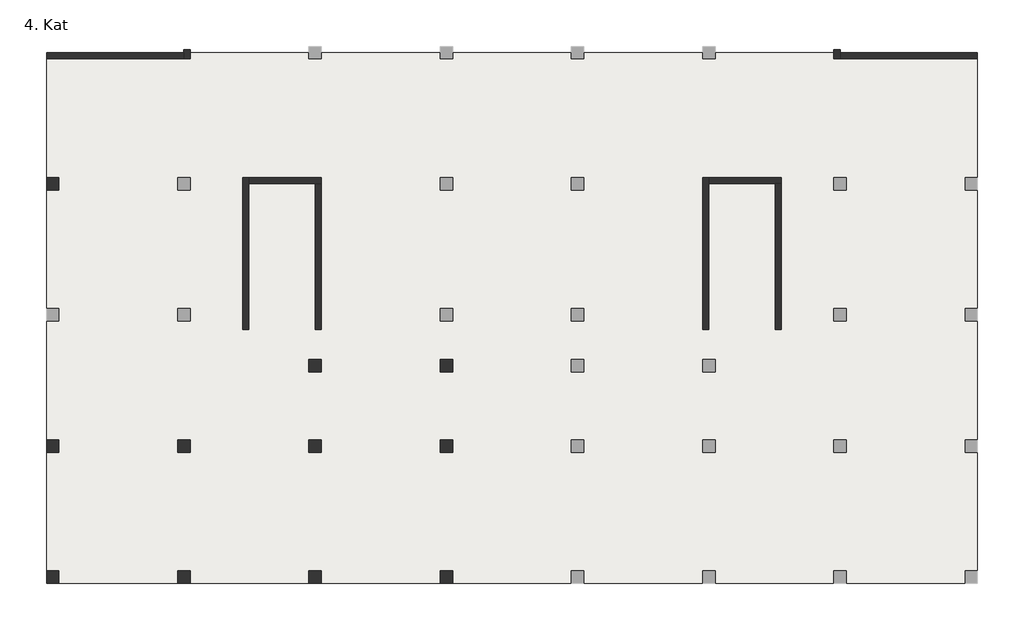
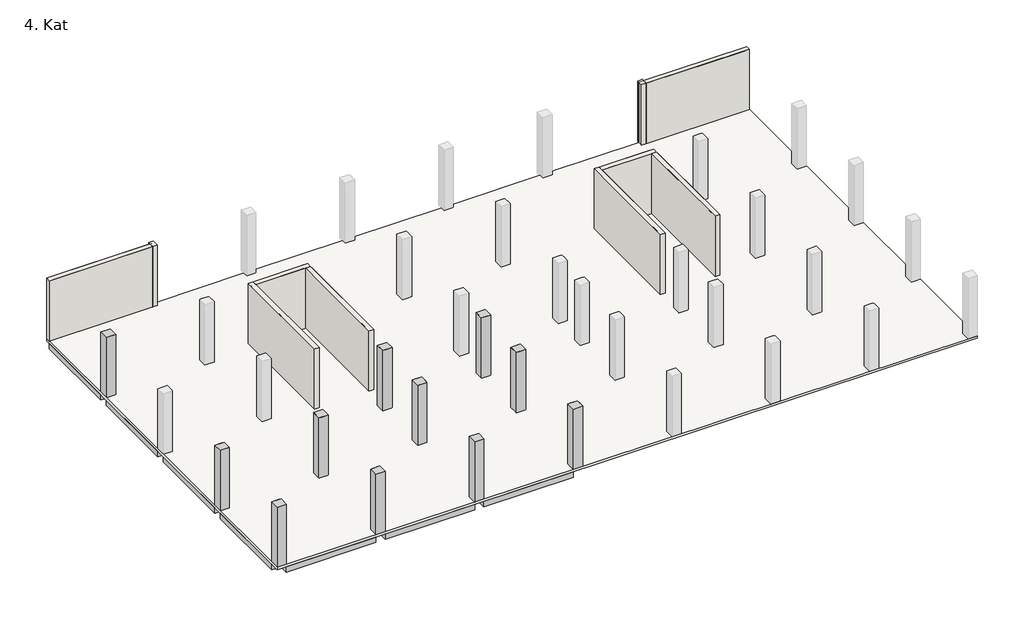
# One storey, part 1 of 2: 22 columns, 20 walls, 10 beams, 1 slab.
"""IFC4 building model written with IfcOpenShell, lengths in millimetres."""

from ifc_helpers import new_model, si_unit, frame, origin, place, context, project, spatial, polyline, outline, extrude, faceted_brep, element, save

model = new_model("IFC4")

# Units and contexts
model_context = context("Model", 3, world=origin())
ifc_project = project(units=[si_unit("LENGTHUNIT", "METRE", prefix="MILLI")], contexts=[model_context])

# Site, building, storey
site = spatial("IfcSite", under=ifc_project)
building = spatial("IfcBuilding", under=site)
storey = spatial("IfcBuildingStorey", under=building, Name="4. Kat", Elevation=21000.0)

# Beams
placement = place(None, origin())
element("IfcBeam", 1, ObjectType="M_Concrete-Rectangular Beam : 60x70cm kiriş", at=placement, inside=storey, context=model_context, shape_type="SweptSolid", body=[
    extrude(outline(polyline([(199.9996111, 8099.9999582), (199.9996111, 399.9999408), (-400.0003889, 399.9999408), (-400.0003889, 8099.9999582), (199.9996111, 8099.9999582)])), frame((0.0, 0.0, 20300.0), z_axis=(0.0, 0.0, 1.0), x_axis=(1.0, 0.0, 0.0)), (0.0, 0.0, 1.0), 500.0),
])
element("IfcBeam", 2, ObjectType="M_Concrete-Rectangular Beam : 60x70cm kiriş", at=placement, inside=storey, context=model_context, shape_type="SweptSolid", body=[
    extrude(outline(polyline([(199.9996411, 16599.9999423), (199.9996411, 8899.9999251), (-400.0003589, 8899.9999251), (-400.0003589, 16599.9999423), (199.9996411, 16599.9999423)])), frame((0.0, 0.0, 20300.0), z_axis=(0.0, 0.0, 1.0), x_axis=(1.0, 0.0, 0.0)), (0.0, 0.0, 1.0), 500.0),
])
element("IfcBeam", 3, ObjectType="M_Concrete-Rectangular Beam : 60x70cm kiriş", at=placement, inside=storey, context=model_context, shape_type="Brep", body=[
    faceted_brep([(199.9994072, 17399.9999423, 20300.0), (199.9994072, 23399.9999249, 20300.0), (199.9994072, 23899.9999249, 20300.0), (199.9994072, 25099.999926, 20300.0), (199.9994072, 25099.999926, 20800.0), (199.9994072, 23899.9999249, 20800.0), (199.9994072, 23399.9999249, 20800.0), (199.9994072, 17399.9999423, 20800.0), (-400.0005928, 17399.9999423, 20300.0), (-400.0005928, 25099.999926, 20300.0), (-400.0005928, 17399.9999423, 20800.0), (-400.0005928, 25099.999926, 20800.0)], [[[0, 1, 2, 3, 4, 5, 6, 7]], [[3, 2, 1, 0, 8, 9]], [[9, 8, 10, 11]], [[7, 6, 5, 4, 11, 10]], [[8, 0, 7, 10]], [[3, 9, 11, 4]]]),
])
element("IfcBeam", 4, ObjectType="M_Concrete-Rectangular Beam : 60x70cm kiriş", at=placement, inside=storey, context=model_context, shape_type="SweptSolid", body=[
    extrude(outline(polyline([(199.9994681, 25899.9999188), (-400.0005319, 25899.9999188), (-400.0005319, 33600.0004302), (199.9994681, 33600.0004302), (199.9994681, 25899.9999188)])), frame((0.0, 0.0, 20300.0), z_axis=(0.0, 0.0, 1.0), x_axis=(1.0, 0.0, 0.0)), (0.0, 0.0, 1.0), 500.0),
])
element("IfcBeam", 5, ObjectType="M_Concrete-Rectangular Beam : 60x70cm kiriş", at=placement, inside=storey, context=model_context, shape_type="SweptSolid", body=[
    extrude(outline(polyline([(8099.9996095, -400.0004808), (399.9996111, -400.0004808), (399.9996111, 199.9995192), (8099.9996095, 199.9995192), (8099.9996095, -400.0004808)])), frame((0.0, 0.0, 20300.0), z_axis=(0.0, 0.0, 1.0), x_axis=(1.0, 0.0, 0.0)), (0.0, 0.0, 1.0), 500.0),
])
element("IfcBeam", 6, ObjectType="M_Concrete-Rectangular Beam : 60x70cm kiriş", at=placement, inside=storey, context=model_context, shape_type="SweptSolid", body=[
    extrude(outline(polyline([(16599.9996095, -400.0000423), (8899.9996095, -400.0000423), (8899.9996095, 199.9999577), (16599.9996095, 199.9999577), (16599.9996095, -400.0000423)])), frame((0.0, 0.0, 20300.0), z_axis=(0.0, 0.0, 1.0), x_axis=(1.0, 0.0, 0.0)), (0.0, 0.0, 1.0), 500.0),
])
element("IfcBeam", 7, ObjectType="M_Concrete-Rectangular Beam : 60x70cm kiriş", at=placement, inside=storey, context=model_context, shape_type="SweptSolid", body=[
    extrude(outline(polyline([(25099.9996096, -399.9996163), (17399.9993907, -399.9996163), (17399.9993907, 200.0003837), (25099.9996096, 200.0003837), (25099.9996096, -399.9996163)])), frame((0.0, 0.0, 20300.0), z_axis=(0.0, 0.0, 1.0), x_axis=(1.0, 0.0, 0.0)), (0.0, 0.0, 1.0), 500.0),
])
element("IfcBeam", 8, ObjectType="M_Concrete-Rectangular Beam : 60x70cm kiriş", at=placement, inside=storey, context=model_context, shape_type="SweptSolid", body=[
    extrude(outline(polyline([(8899.9996095, 8100.0003637), (8899.9996095, 399.9999384), (8299.9996095, 399.9999384), (8299.9996095, 8100.0003637), (8899.9996095, 8100.0003637)])), frame((0.0, 0.0, 20300.0), z_axis=(0.0, 0.0, 1.0), x_axis=(1.0, 0.0, 0.0)), (0.0, 0.0, 1.0), 500.0),
])
element("IfcBeam", 9, ObjectType="M_Concrete-Rectangular Beam : 60x70cm kiriş", at=placement, inside=storey, context=model_context, shape_type="Brep", body=[
    faceted_brep([(8899.9996095, 8900.0003637, 20300.0), (8899.9996095, 13300.0003638, 20300.0), (8899.9996095, 13700.0003638, 20300.0), (8899.9996095, 16599.9999418, 20300.0), (8899.9996095, 16599.9999418, 20800.0), (8899.9996095, 13700.0003638, 20800.0), (8899.9996095, 13300.0003638, 20800.0), (8899.9996095, 8900.0003637, 20800.0), (8299.9996095, 8900.0003637, 20300.0), (8299.9996095, 16599.9999418, 20300.0), (8299.9996095, 8900.0003637, 20800.0), (8299.9996095, 16599.9999418, 20800.0)], [[[0, 1, 2, 3, 4, 5, 6, 7]], [[3, 2, 1, 0, 8, 9]], [[9, 8, 10, 11]], [[7, 6, 5, 4, 11, 10]], [[8, 0, 7, 10]], [[3, 9, 11, 4]]]),
])
element("IfcBeam", 10, ObjectType="M_Concrete-Rectangular Beam : 60x70cm kiriş", at=placement, inside=storey, context=model_context, shape_type="SweptSolid", body=[
    extrude(outline(polyline([(8099.9997451, 8200.0009197), (399.9996411, 8200.0009197), (399.9996411, 8800.0009197), (8099.9997451, 8800.0009197), (8099.9997451, 8200.0009197)])), frame((0.0, 0.0, 20300.0), z_axis=(0.0, 0.0, 1.0), x_axis=(1.0, 0.0, 0.0)), (0.0, 0.0, 1.0), 500.0),
])

# Columns
element("IfcColumn", 11, ObjectType="M_Concrete-Rectangular-Column : 80x80cm kolon", at=placement, inside=storey, context=model_context, shape_type="SweptSolid", body=[
    extrude(outline(polyline([(400.0000836, 400.0009197), (400.0000836, -399.9990803), (-399.9999164, -399.9990803), (-399.9999164, 400.0009197), (400.0000836, 400.0009197)])), frame((0.0, 0.0, 21000.0), z_axis=(0.0, 0.0, 1.0), x_axis=(1.0, 0.0, 0.0)), (0.0, 0.0, 1.0), 5500.0),
])
element("IfcColumn", 12, ObjectType="M_Concrete-Rectangular-Column : 80x80cm kolon", at=placement, inside=storey, context=model_context, shape_type="SweptSolid", body=[
    extrude(outline(polyline([(8899.9993907, 400.0009197), (8899.9993907, -399.9990803), (8099.9993907, -399.9990803), (8099.9993907, 400.0009197), (8899.9993907, 400.0009197)])), frame((0.0, 0.0, 21000.0), z_axis=(0.0, 0.0, 1.0), x_axis=(1.0, 0.0, 0.0)), (0.0, 0.0, 1.0), 5500.0),
])
element("IfcColumn", 13, ObjectType="M_Concrete-Rectangular-Column : 80x80cm kolon", at=placement, inside=storey, context=model_context, shape_type="SweptSolid", body=[
    extrude(outline(polyline([(400.0000836, 8900.0009197), (400.0000836, 8100.0009197), (-399.9999164, 8100.0009197), (-399.9999164, 8900.0009197), (400.0000836, 8900.0009197)])), frame((0.0, 0.0, 21000.0), z_axis=(0.0, 0.0, 1.0), x_axis=(1.0, 0.0, 0.0)), (0.0, 0.0, 1.0), 5500.0),
])
element("IfcColumn", 14, ObjectType="M_Concrete-Rectangular-Column : 80x80cm kolon", at=placement, inside=storey, context=model_context, shape_type="SweptSolid", body=[
    extrude(outline(polyline([(8899.9993907, 8900.0009197), (8899.9993907, 8100.0009197), (8099.9993907, 8100.0009197), (8099.9993907, 8900.0009197), (8899.9993907, 8900.0009197)])), frame((0.0, 0.0, 21000.0), z_axis=(0.0, 0.0, 1.0), x_axis=(1.0, 0.0, 0.0)), (0.0, 0.0, 1.0), 5500.0),
])
element("IfcColumn", 15, ObjectType="M_Concrete-Rectangular-Column : 80x80cm kolon", at=placement, inside=storey, context=model_context, shape_type="SweptSolid", body=[
    extrude(outline(polyline([(399.9996699, 25899.9999188), (399.9996699, 25099.9999188), (-400.0003301, 25099.9999188), (-400.0003301, 25899.9999188), (399.9996699, 25899.9999188)])), frame((0.0, 0.0, 21000.0), z_axis=(0.0, 0.0, 1.0), x_axis=(1.0, 0.0, 0.0)), (0.0, 0.0, 1.0), 5500.0),
])
element("IfcColumn", 16, ObjectType="M_Concrete-Rectangular-Column : 80x80cm kolon", at=placement, inside=storey, context=model_context, shape_type="SweptSolid", body=[
    extrude(outline(polyline([(17399.9993907, 8900.0009197), (17399.9993907, 8100.0009197), (16599.9993907, 8100.0009197), (16599.9993907, 8900.0009197), (17399.9993907, 8900.0009197)])), frame((0.0, 0.0, 21000.0), z_axis=(0.0, 0.0, 1.0), x_axis=(1.0, 0.0, 0.0)), (0.0, 0.0, 1.0), 5500.0),
])
element("IfcColumn", 17, ObjectType="M_Concrete-Rectangular-Column : 80x80cm kolon", at=placement, inside=storey, context=model_context, shape_type="SweptSolid", body=[
    extrude(outline(polyline([(25899.9993907, 8900.0009197), (25899.9993907, 8100.0009197), (25099.9993907, 8100.0009197), (25099.9993907, 8900.0009197), (25899.9993907, 8900.0009197)])), frame((0.0, 0.0, 21000.0), z_axis=(0.0, 0.0, 1.0), x_axis=(1.0, 0.0, 0.0)), (0.0, 0.0, 1.0), 5500.0),
])
element("IfcColumn", 18, ObjectType="M_Concrete-Rectangular-Column : 80x80cm kolon", at=placement, inside=storey, context=model_context, shape_type="SweptSolid", body=[
    extrude(outline(polyline([(25899.9993907, 400.0009197), (25899.9993907, -399.9990803), (25099.9993907, -399.9990803), (25099.9993907, 400.0009197), (25899.9993907, 400.0009197)])), frame((0.0, 0.0, 21000.0), z_axis=(0.0, 0.0, 1.0), x_axis=(1.0, 0.0, 0.0)), (0.0, 0.0, 1.0), 5500.0),
])
element("IfcColumn", 19, ObjectType="M_Concrete-Rectangular-Column : 80x80cm kolon", at=placement, inside=storey, context=model_context, shape_type="SweptSolid", body=[
    extrude(outline(polyline([(17399.9993907, 400.0009197), (17399.9993907, -399.9990803), (16599.9993907, -399.9990803), (16599.9993907, 400.0009197), (17399.9993907, 400.0009197)])), frame((0.0, 0.0, 21000.0), z_axis=(0.0, 0.0, 1.0), x_axis=(1.0, 0.0, 0.0)), (0.0, 0.0, 1.0), 5500.0),
])
element("IfcColumn", 20, ObjectType="M_Concrete-Rectangular-Column : 80x80cm kolon", at=placement, inside=storey, context=model_context, shape_type="SweptSolid", body=[
    extrude(outline(polyline([(25899.9993907, 14100.0003995), (25899.9993907, 13300.0003995), (25099.9993907, 13300.0003995), (25099.9993907, 14100.0003995), (25899.9993907, 14100.0003995)])), frame((0.0, 0.0, 21000.0), z_axis=(0.0, 0.0, 1.0), x_axis=(1.0, 0.0, 0.0)), (0.0, 0.0, 1.0), 5500.0),
])
element("IfcColumn", 21, ObjectType="M_Concrete-Rectangular-Column : 80x80cm kolon", at=placement, inside=storey, context=model_context, shape_type="SweptSolid", body=[
    extrude(outline(polyline([(17399.9993907, 14099.9451047), (17399.9993907, 13299.9451047), (16599.9993907, 13299.9451047), (16599.9993907, 14099.9451047), (17399.9993907, 14099.9451047)])), frame((0.0, 0.0, 21000.0), z_axis=(0.0, 0.0, 1.0), x_axis=(1.0, 0.0, 0.0)), (0.0, 0.0, 1.0), 5500.0),
])
element("IfcColumn", 22, ObjectType="M_Concrete-Rectangular-Column : 80x80cm kolon", at=placement, inside=storey, context=model_context, shape_type="Brep", body=[
    faceted_brep([(400.0000836, 400.0009197, 21000.0), (400.0000836, -399.9990803, 21000.0), (-399.9999164, -399.9990803, 21000.0), (-399.9999164, 400.0009197, 21000.0), (400.0000836, 400.0009197, 26500.0), (400.0000836, 199.9995192, 26500.0), (400.0000836, -399.9990803, 26500.0), (-399.9999164, -399.9990803, 26500.0), (-399.9999164, 400.0009197, 26500.0), (199.9996111, 400.0009197, 26500.0)], [[[0, 1, 2, 3]], [[4, 5, 6, 1, 0]], [[6, 7, 2, 1]], [[7, 8, 3, 2]], [[8, 9, 4, 0, 3]], [[4, 9, 8, 7, 6, 5]]]),
])
element("IfcColumn", 23, ObjectType="M_Concrete-Rectangular-Column : 80x80cm kolon", at=placement, inside=storey, context=model_context, shape_type="Brep", body=[
    faceted_brep([(8899.9993907, 400.0009197, 21000.0), (8899.9993907, -399.9990803, 21000.0), (8099.9993907, -399.9990803, 21000.0), (8099.9993907, 400.0009197, 21000.0), (8899.9993907, 400.0009197, 26500.0), (8899.9993907, 199.9999577, 26500.0), (8899.9993907, -399.9990803, 26500.0), (8099.9993907, -399.9990803, 26500.0), (8099.9993907, 199.9995192, 26500.0), (8099.9993907, 400.0009197, 26500.0), (8299.9996095, 400.0009197, 26500.0)], [[[0, 1, 2, 3]], [[4, 5, 6, 1, 0]], [[6, 7, 2, 1]], [[7, 8, 9, 3, 2]], [[9, 10, 4, 0, 3]], [[4, 10, 9, 8, 7, 6, 5]]]),
])
element("IfcColumn", 24, ObjectType="M_Concrete-Rectangular-Column : 80x80cm kolon", at=placement, inside=storey, context=model_context, shape_type="Brep", body=[
    faceted_brep([(400.0000836, 8900.0009197, 21000.0), (400.0000836, 8100.0009197, 21000.0), (-399.9999164, 8100.0009197, 21000.0), (-399.9999164, 8900.0009197, 21000.0), (400.0000836, 8900.0009197, 26500.0), (400.0000836, 8800.0009197, 26500.0), (400.0000836, 8200.0009197, 26500.0), (400.0000836, 8100.0009197, 26500.0), (199.9996111, 8100.0009197, 26500.0), (-399.9999164, 8100.0009197, 26500.0), (-399.9999164, 8900.0009197, 26500.0), (199.9996411, 8900.0009197, 26500.0)], [[[0, 1, 2, 3]], [[4, 5, 6, 7, 1, 0]], [[7, 8, 9, 2, 1]], [[9, 10, 3, 2]], [[10, 11, 4, 0, 3]], [[4, 11, 10, 9, 8, 7, 6, 5]]]),
])
element("IfcColumn", 25, ObjectType="M_Concrete-Rectangular-Column : 80x80cm kolon", at=placement, inside=storey, context=model_context, shape_type="Brep", body=[
    faceted_brep([(8899.9993907, 8900.0009197, 21000.0), (8899.9993907, 8100.0009197, 21000.0), (8099.9993907, 8100.0009197, 21000.0), (8099.9993907, 8900.0009197, 21000.0), (8899.9993907, 8900.0009197, 26500.0), (8899.9993907, 8800.0009197, 26500.0), (8899.9993907, 8200.0009197, 26500.0), (8899.9993907, 8100.0009197, 26500.0), (8299.9996095, 8100.0009197, 26500.0), (8099.9993907, 8100.0009197, 26500.0), (8099.9993907, 8200.0009197, 26500.0), (8099.9993907, 8800.0009197, 26500.0), (8099.9993907, 8900.0009197, 26500.0), (8299.9996095, 8900.0009197, 26500.0)], [[[0, 1, 2, 3]], [[4, 5, 6, 7, 1, 0]], [[7, 8, 9, 2, 1]], [[9, 10, 11, 12, 3, 2]], [[12, 13, 4, 0, 3]], [[4, 13, 12, 11, 10, 9, 8, 7, 6, 5]]]),
])
element("IfcColumn", 26, ObjectType="M_Concrete-Rectangular-Column : 80x80cm kolon", at=placement, inside=storey, context=model_context, shape_type="Brep", body=[
    faceted_brep([(399.9996699, 25899.9999188, 21000.0), (399.9996699, 25099.9999188, 21000.0), (-400.0003301, 25099.9999188, 21000.0), (-400.0003301, 25899.9999188, 21000.0), (399.9996699, 25899.9999188, 26500.0), (399.9996699, 25299.999992, 26500.0), (399.9996699, 25099.9999188, 26500.0), (199.9994072, 25099.9999188, 26500.0), (-400.0003301, 25099.9999188, 26500.0), (-400.0003301, 25899.9999188, 26500.0), (199.9994681, 25899.9999188, 26500.0)], [[[0, 1, 2, 3]], [[4, 5, 6, 1, 0]], [[6, 7, 8, 2, 1]], [[8, 9, 3, 2]], [[9, 10, 4, 0, 3]], [[4, 10, 9, 8, 7, 6, 5]]]),
])
element("IfcColumn", 27, ObjectType="M_Concrete-Rectangular-Column : 80x80cm kolon", at=placement, inside=storey, context=model_context, shape_type="Brep", body=[
    faceted_brep([(17399.9993907, 8900.0009197, 21000.0), (17399.9993907, 8100.0009197, 21000.0), (16599.9993907, 8100.0009197, 21000.0), (16599.9993907, 8900.0009197, 21000.0), (17399.9993907, 8900.0009197, 26500.0), (17399.9993907, 8800.0009197, 26500.0), (17399.9993907, 8200.0009197, 26500.0), (17399.9993907, 8100.0009197, 26500.0), (16799.9997451, 8100.0009197, 26500.0), (16599.9993907, 8100.0009197, 26500.0), (16599.9993907, 8200.0009197, 26500.0), (16599.9993907, 8800.0009197, 26500.0), (16599.9993907, 8900.0009197, 26500.0), (16799.9997293, 8900.0009197, 26500.0)], [[[0, 1, 2, 3]], [[4, 5, 6, 7, 1, 0]], [[7, 8, 9, 2, 1]], [[9, 10, 11, 12, 3, 2]], [[12, 13, 4, 0, 3]], [[4, 13, 12, 11, 10, 9, 8, 7, 6, 5]]]),
])
element("IfcColumn", 28, ObjectType="M_Concrete-Rectangular-Column : 80x80cm kolon", at=placement, inside=storey, context=model_context, shape_type="Brep", body=[
    faceted_brep([(25899.9993907, 8900.0009197, 21000.0), (25899.9993907, 8100.0009197, 21000.0), (25099.9993907, 8100.0009197, 21000.0), (25099.9993907, 8900.0009197, 21000.0), (25899.9993907, 8900.0009197, 26500.0), (25899.9993907, 8800.0009197, 26500.0), (25899.9993907, 8200.0009197, 26500.0), (25899.9993907, 8100.0009197, 26500.0), (25299.9997233, 8100.0009197, 26500.0), (25099.9993907, 8100.0009197, 26500.0), (25099.9993907, 8200.0009197, 26500.0), (25099.9993907, 8800.0009197, 26500.0), (25099.9993907, 8900.0009197, 26500.0), (25299.9997233, 8900.0009197, 26500.0)], [[[0, 1, 2, 3]], [[4, 5, 6, 7, 1, 0]], [[7, 8, 9, 2, 1]], [[9, 10, 11, 12, 3, 2]], [[12, 13, 4, 0, 3]], [[4, 13, 12, 11, 10, 9, 8, 7, 6, 5]]]),
])
element("IfcColumn", 29, ObjectType="M_Concrete-Rectangular-Column : 80x80cm kolon", at=placement, inside=storey, context=model_context, shape_type="Brep", body=[
    faceted_brep([(25899.9993907, 400.0009197, 21000.0), (25899.9993907, -399.9990803, 21000.0), (25099.9993907, -399.9990803, 21000.0), (25099.9993907, 400.0009197, 21000.0), (25899.9993907, 400.0009197, 26500.0), (25899.9993907, 200.0003118, 26500.0), (25899.9993907, -399.9990803, 26500.0), (25099.9993907, -399.9990803, 26500.0), (25099.9993907, 200.0003837, 26500.0), (25099.9993907, 400.0009197, 26500.0), (25299.9997233, 400.0009197, 26500.0)], [[[0, 1, 2, 3]], [[4, 5, 6, 1, 0]], [[6, 7, 2, 1]], [[7, 8, 9, 3, 2]], [[9, 10, 4, 0, 3]], [[4, 10, 9, 8, 7, 6, 5]]]),
])
element("IfcColumn", 30, ObjectType="M_Concrete-Rectangular-Column : 80x80cm kolon", at=placement, inside=storey, context=model_context, shape_type="Brep", body=[
    faceted_brep([(17399.9993907, 400.0009197, 21000.0), (17399.9993907, -399.9990803, 21000.0), (16599.9993907, -399.9990803, 21000.0), (16599.9993907, 400.0009197, 21000.0), (17399.9993907, 400.0009197, 26500.0), (17399.9993907, 200.0003837, 26500.0), (17399.9993907, -399.9990803, 26500.0), (16599.9993907, -399.9990803, 26500.0), (16599.9993907, 199.9999577, 26500.0), (16599.9993907, 400.0009197, 26500.0), (16799.9997451, 400.0009197, 26500.0)], [[[0, 1, 2, 3]], [[4, 5, 6, 1, 0]], [[6, 7, 2, 1]], [[7, 8, 9, 3, 2]], [[9, 10, 4, 0, 3]], [[4, 10, 9, 8, 7, 6, 5]]]),
])
element("IfcColumn", 31, ObjectType="M_Concrete-Rectangular-Column : 80x80cm kolon", at=placement, inside=storey, context=model_context, shape_type="Brep", body=[
    faceted_brep([(25899.9993907, 14100.0003995, 21000.0), (25899.9993907, 13300.0003995, 21000.0), (25099.9993907, 13300.0003995, 21000.0), (25099.9993907, 14100.0003995, 21000.0), (25899.9993907, 14100.0003995, 26500.0), (25899.9993907, 13700.0003995, 26500.0), (25899.9993907, 13300.0003995, 26500.0), (25899.9993907, 13300.0003995, 25800.0), (25299.9997233, 13300.0003995, 26500.0), (25099.9993907, 13300.0003995, 26500.0), (25099.9993907, 13300.0003995, 25800.0), (25099.9993907, 13700.0003995, 26500.0), (25099.9993907, 14100.0003995, 26500.0), (25299.9997233, 14100.0003995, 26500.0)], [[[0, 1, 2, 3]], [[4, 5, 6, 7, 1, 0]], [[6, 8, 9, 10, 2, 1, 7]], [[9, 11, 12, 3, 2, 10]], [[12, 13, 4, 0, 3]], [[4, 13, 12, 11, 9, 8, 6, 5]]]),
])
element("IfcColumn", 32, ObjectType="M_Concrete-Rectangular-Column : 80x80cm kolon", at=placement, inside=storey, context=model_context, shape_type="Brep", body=[
    faceted_brep([(17399.9993907, 14099.9451047, 21000.0), (17399.9993907, 13299.9451047, 21000.0), (16599.9993907, 13299.9451047, 21000.0), (16599.9993907, 14099.9451047, 21000.0), (17399.9993907, 14099.9451047, 26500.0), (17399.9993907, 13700.0003995, 26500.0), (17399.9993907, 13299.9451047, 26500.0), (16799.9997293, 13299.9451047, 26500.0), (16599.9993907, 13299.9451047, 26500.0), (16599.9993907, 13700.0003638, 26500.0), (16599.9993907, 14099.9451047, 26500.0), (16999.9995362, 14099.9451047, 26500.0)], [[[0, 1, 2, 3]], [[4, 5, 6, 1, 0]], [[6, 7, 8, 2, 1]], [[8, 9, 10, 3, 2]], [[10, 11, 4, 0, 3]], [[4, 11, 10, 9, 8, 7, 6, 5]]]),
])

# Slab
element("IfcSlab", 33, ObjectType="20 cm döşeme", at=placement, inside=storey, context=model_context, shape_type="Brep", body=[
    faceted_brep([(59899.9997758, 34000.0004302, 20800.0), (59899.9997758, 16600.0009197, 20800.0), (59899.9997758, 8900.0009197, 20800.0), (59899.9997758, -399.9995292, 20800.0), (-400.0005319, -399.9995292, 20800.0), (-400.0005319, 25899.9999188, 20800.0), (-400.0005319, 33600.0004302, 20800.0), (-400.0005319, 34000.0004302, 20800.0), (8899.9993907, 34000.0004302, 20800.0), (16599.9993907, 34000.0004302, 20800.0), (17399.9993907, 34000.0004302, 20800.0), (25099.9993907, 34000.0004302, 20800.0), (25899.9993907, 34000.0004302, 20800.0), (33599.9993907, 34000.0004302, 20800.0), (34399.9993907, 34000.0004302, 20800.0), (42099.9993899, 34000.0004302, 20800.0), (42899.999681, 34000.0004302, 20800.0), (50599.9994944, 34000.0004302, 20800.0), (59899.9997758, 34000.0004302, 21000.0), (51199.9994348, 34000.0004302, 21000.0), (50999.9994944, 34000.0004302, 21000.0), (50599.9994944, 34000.0004302, 21000.0), (42899.999681, 34000.0004302, 21000.0), (42099.9993899, 34000.0004302, 21000.0), (34399.9993907, 34000.0004302, 21000.0), (33599.9993907, 34000.0004302, 21000.0), (25899.9993907, 34000.0004302, 21000.0), (25099.9993907, 34000.0004302, 21000.0), (17399.9993907, 34000.0004302, 21000.0), (16599.9993907, 34000.0004302, 21000.0), (8899.9995273, 34000.0004302, 21000.0), (8499.9995273, 34000.0004302, 21000.0), (8299.9993907, 34000.0004302, 21000.0), (-400.0005319, 34000.0004302, 21000.0), (-400.0005319, -399.9995292, 21000.0), (59899.9997758, -399.9995292, 21000.0), (59899.9997758, 8200.0009197, 21000.0), (59899.9997758, 8800.0009197, 21000.0), (59899.9997758, 17000.0009197, 21000.0)], [[[0, 1, 2, 3, 4, 5, 6, 7, 8, 9, 10, 11, 12, 13, 14, 15, 16, 17]], [[18, 19, 20, 21, 22, 23, 24, 25, 26, 27, 28, 29, 30, 31, 32, 33, 34, 35, 36, 37, 38]], [[3, 2, 1, 0, 18, 38, 37, 36, 35]], [[4, 3, 35, 34]], [[7, 6, 5, 4, 34, 33]], [[0, 17, 16, 15, 14, 13, 12, 11, 10, 9, 8, 7, 33, 32, 31, 30, 29, 28, 27, 26, 25, 24, 23, 22, 21, 20, 19, 18]]]),
])

# Walls
element("IfcWall", 34, ObjectType="40cm perde duvar", at=placement, inside=storey, context=model_context, shape_type="SweptSolid", body=[
    extrude(outline(polyline([(8499.9995273, 33600.0004302), (-400.0005319, 33600.0004302), (-400.0005319, 34000.0004302), (8499.9995273, 34000.0004302), (8499.9995273, 33600.0004302)])), frame((0.0, 0.0, 21000.0), z_axis=(0.0, 0.0, 1.0), x_axis=(1.0, 0.0, 0.0)), (0.0, 0.0, 1.0), 5500.0),
])
element("IfcWall", 35, ObjectType="40cm perde duvar", at=placement, inside=storey, context=model_context, shape_type="SweptSolid", body=[
    extrude(outline(polyline([(8899.9995273, 34200.0004302), (8899.9995273, 34000.0004302), (8499.9995273, 34000.0004302), (8499.9995273, 34200.0004302), (8899.9995273, 34200.0004302)])), frame((0.0, 0.0, 21000.0), z_axis=(0.0, 0.0, 1.0), x_axis=(1.0, 0.0, 0.0)), (0.0, 0.0, 1.0), 5500.0),
])
element("IfcWall", 36, ObjectType="40cm perde duvar", at=placement, inside=storey, context=model_context, shape_type="Brep", body=[
    faceted_brep([(12700.0064017, 16050.000156, 21000.0), (12700.0064017, 25500.0003816, 21000.0), (12700.0064017, 25900.0003816, 21000.0), (12700.0064017, 25900.0003816, 26500.0), (12700.0064017, 25500.0003816, 26500.0), (12700.0064017, 16050.000156, 26500.0), (12700.0064017, 16050.000156, 25800.0), (12300.0064017, 16050.000156, 21000.0), (12300.0064017, 16050.000156, 25800.0), (12300.0064017, 16050.000156, 26500.0), (12300.0064017, 25900.0003816, 26500.0), (12300.0064017, 25900.0003816, 21000.0)], [[[0, 1, 2, 3, 4, 5, 6]], [[7, 8, 9, 10, 11]], [[2, 1, 0, 7, 11]], [[5, 4, 3, 10, 9]], [[0, 6, 5, 9, 8, 7]], [[3, 2, 11, 10]]]),
])
element("IfcWall", 37, ObjectType="40cm perde duvar", at=placement, inside=storey, context=model_context, shape_type="Brep", body=[
    faceted_brep([(12700.0064017, 25500.0003816, 21000.0), (16999.9995362, 25500.0003816, 21000.0), (17399.9995362, 25500.0003816, 21000.0), (17399.9995362, 25500.0003816, 26500.0), (16999.9995362, 25500.0003816, 26500.0), (12700.0064017, 25500.0003816, 26500.0), (12700.0064017, 25900.0003816, 21000.0), (12700.0064017, 25900.0003816, 26500.0), (17399.9995362, 25900.0003816, 26500.0), (17399.9995362, 25900.0003816, 21000.0)], [[[0, 1, 2, 3, 4, 5]], [[6, 7, 8, 9]], [[2, 1, 0, 6, 9]], [[5, 4, 3, 8, 7]], [[0, 5, 7, 6]], [[3, 2, 9, 8]]]),
])
element("IfcWall", 38, ObjectType="40cm perde duvar", at=placement, inside=storey, context=model_context, shape_type="Brep", body=[
    faceted_brep([(16999.9995362, 25500.0003816, 21000.0), (16999.9995362, 16050.0003816, 21000.0), (16999.9995362, 16050.0003816, 25800.0), (16999.9995362, 16050.0003816, 26500.0), (16999.9995362, 25500.0003816, 26500.0), (17399.9995362, 25500.0003816, 21000.0), (17399.9995362, 25500.0003816, 26500.0), (17399.9995362, 16050.0003816, 26500.0), (17399.9995362, 16050.0003816, 25800.0), (17399.9995362, 16050.0003816, 21000.0)], [[[0, 1, 2, 3, 4]], [[5, 6, 7, 8, 9]], [[1, 0, 5, 9]], [[3, 2, 1, 9, 8, 7]], [[4, 3, 7, 6]], [[0, 4, 6, 5]]]),
])
element("IfcWall", 39, ObjectType="40cm perde duvar", at=placement, inside=storey, context=model_context, shape_type="Brep", body=[
    faceted_brep([(42499.9995162, 16050.0004138, 21000.0), (42499.9995162, 25500.0004459, 21000.0), (42499.9995162, 25900.0004459, 21000.0), (42499.9995162, 25900.0004459, 26500.0), (42499.9995162, 25500.0004459, 26500.0), (42499.9995162, 16050.0004138, 26500.0), (42499.9995162, 16050.0004138, 25800.0), (42099.9995162, 16050.0004138, 21000.0), (42099.9995162, 16050.0004138, 25800.0), (42099.9995162, 16050.0004138, 26500.0), (42099.9995162, 25900.0004459, 26500.0), (42099.9995162, 25900.0004459, 21000.0)], [[[0, 1, 2, 3, 4, 5, 6]], [[7, 8, 9, 10, 11]], [[2, 1, 0, 7, 11]], [[5, 4, 3, 10, 9]], [[0, 6, 5, 9, 8, 7]], [[3, 2, 11, 10]]]),
])
element("IfcWall", 40, ObjectType="40cm perde duvar", at=placement, inside=storey, context=model_context, shape_type="Brep", body=[
    faceted_brep([(42499.9995162, 25500.0004459, 21000.0), (46799.999381, 25500.0004459, 21000.0), (47199.999381, 25500.0004459, 21000.0), (47199.999381, 25500.0004459, 26500.0), (46799.999381, 25500.0004459, 26500.0), (42499.9995162, 25500.0004459, 26500.0), (42499.9995162, 25900.0004459, 21000.0), (42499.9995162, 25900.0004459, 26500.0), (47199.999381, 25900.0004459, 26500.0), (47199.999381, 25900.0004459, 21000.0)], [[[0, 1, 2, 3, 4, 5]], [[6, 7, 8, 9]], [[2, 1, 0, 6, 9]], [[5, 4, 3, 8, 7]], [[0, 5, 7, 6]], [[3, 2, 9, 8]]]),
])
element("IfcWall", 41, ObjectType="40cm perde duvar", at=placement, inside=storey, context=model_context, shape_type="Brep", body=[
    faceted_brep([(46799.999381, 25500.0004459, 21000.0), (46799.999381, 16050.0004138, 21000.0), (46799.999381, 16050.0004138, 25800.0), (46799.999381, 16050.0004138, 26500.0), (46799.999381, 25500.0004459, 26500.0), (47199.999381, 25500.0004459, 21000.0), (47199.999381, 25500.0004459, 26500.0), (47199.999381, 16050.0004138, 26500.0), (47199.999381, 16050.0004138, 25800.0), (47199.999381, 16050.0004138, 21000.0)], [[[0, 1, 2, 3, 4]], [[5, 6, 7, 8, 9]], [[1, 0, 5, 9]], [[3, 2, 1, 9, 8, 7]], [[4, 3, 7, 6]], [[0, 4, 6, 5]]]),
])
element("IfcWall", 42, ObjectType="40cm perde duvar", at=placement, inside=storey, context=model_context, shape_type="Brep", body=[
    faceted_brep([(50599.9994944, 34193.7257565, 21000.0), (50599.9994944, 33600.0004303, 21000.0), (50599.9994944, 33600.0004303, 26500.0), (50599.9994944, 34193.7257565, 26500.0), (50999.9994944, 34193.7257565, 21000.0), (50999.9994944, 34193.7257565, 26500.0), (50999.9994944, 34000.0004303, 26500.0), (50999.9994944, 33600.0004303, 26500.0), (50999.9994944, 33600.0004303, 21000.0), (50999.9994944, 34000.0004303, 21000.0)], [[[0, 1, 2, 3]], [[4, 5, 6, 7, 8, 9]], [[1, 0, 4, 9, 8]], [[3, 2, 7, 6, 5]], [[0, 3, 5, 4]], [[2, 1, 8, 7]]]),
])
element("IfcWall", 43, ObjectType="40cm perde duvar", at=placement, inside=storey, context=model_context, shape_type="SweptSolid", body=[
    extrude(outline(polyline([(59899.9999497, 33600.0004303), (50999.9994944, 33600.0004303), (50999.9994944, 34000.0004303), (59899.9999497, 34000.0004303), (59899.9999497, 33600.0004303)])), frame((0.0, 0.0, 21000.0), z_axis=(0.0, 0.0, 1.0), x_axis=(1.0, 0.0, 0.0)), (0.0, 0.0, 1.0), 5500.0),
])
element("IfcWall", 44, ObjectType="40cm perde duvar", at=placement, inside=storey, context=model_context, shape_type="Brep", body=[
    faceted_brep([(-400.0005319, 33600.0004302, 21000.0), (8499.9995273, 33600.0004302, 21000.0), (8499.9995273, 33600.0004302, 26500.0), (8299.9993907, 33600.0004302, 26500.0), (199.9994681, 33600.0004302, 26500.0), (-400.0005319, 33600.0004302, 26500.0), (-400.0005319, 33600.0004302, 25800.0), (-400.0005319, 34000.0004302, 21000.0), (-400.0005319, 34000.0004302, 26500.0), (8299.9993907, 34000.0004302, 26500.0), (8499.9995273, 34000.0004302, 26500.0), (8499.9995273, 34000.0004302, 25800.0), (8499.9995273, 34000.0004302, 21000.0)], [[[0, 1, 2, 3, 4, 5, 6]], [[7, 8, 9, 10, 11, 12]], [[1, 0, 7, 12]], [[5, 4, 3, 2, 10, 9, 8]], [[0, 6, 5, 8, 7]], [[2, 1, 12, 11, 10]]]),
])
element("IfcWall", 45, ObjectType="40cm perde duvar", at=placement, inside=storey, context=model_context, shape_type="Brep", body=[
    faceted_brep([(8899.9995273, 33600.0004302, 21000.0), (8899.9995273, 34200.0004302, 21000.0), (8899.9995273, 34200.0004302, 26500.0), (8899.9995273, 33600.0004302, 26500.0), (8499.9995273, 33600.0004302, 21000.0), (8499.9995273, 33600.0004302, 26500.0), (8499.9995273, 34000.0004302, 26500.0), (8499.9995273, 34200.0004302, 26500.0), (8499.9995273, 34200.0004302, 21000.0), (8499.9995273, 34000.0004302, 21000.0)], [[[0, 1, 2, 3]], [[4, 5, 6, 7, 8, 9]], [[1, 0, 4, 9, 8]], [[2, 1, 8, 7]], [[3, 2, 7, 6, 5]], [[0, 3, 5, 4]]]),
])
element("IfcWall", 46, ObjectType="40cm perde duvar", at=placement, inside=storey, context=model_context, shape_type="Brep", body=[
    faceted_brep([(12700.0064017, 16050.000156, 21000.0), (12700.0064017, 25500.0003816, 21000.0), (12700.0064017, 25500.0003816, 26500.0), (12700.0064017, 17400.0003638, 26500.0), (12700.0064017, 17000.0003638, 26500.0), (12700.0064017, 16350.0003638, 26500.0), (12700.0064017, 16050.000156, 26500.0), (12700.0064017, 16050.000156, 25800.0), (12300.0064017, 16050.000156, 21000.0), (12300.0064017, 16050.000156, 25800.0), (12300.0064017, 16050.000156, 26500.0), (12300.0064017, 16800.0003643, 26500.0), (12300.0064017, 17400.0003643, 26500.0), (12300.0064017, 25299.9999925, 26500.0), (12300.0064017, 25500.0003816, 26500.0), (12300.0064017, 25500.0003816, 21000.0)], [[[0, 1, 2, 3, 4, 5, 6, 7]], [[8, 9, 10, 11, 12, 13, 14, 15]], [[1, 0, 8, 15]], [[6, 5, 4, 3, 2, 14, 13, 12, 11, 10]], [[0, 7, 6, 10, 9, 8]], [[2, 1, 15, 14]]]),
])
element("IfcWall", 47, ObjectType="40cm perde duvar", at=placement, inside=storey, context=model_context, shape_type="Brep", body=[
    faceted_brep([(12700.0064017, 25500.0003816, 21000.0), (16999.9995362, 25500.0003816, 21000.0), (16999.9995362, 25500.0003816, 25800.0), (16999.9995362, 25500.0003816, 26500.0), (16799.9996817, 25500.0003816, 26500.0), (12700.0064017, 25500.0003816, 26500.0), (12700.0064017, 25900.0003816, 21000.0), (12700.0064017, 25900.0003816, 26500.0), (16799.9996817, 25900.0003816, 26500.0), (16999.9995362, 25900.0003816, 26500.0), (16999.9995362, 25900.0003816, 21000.0)], [[[0, 1, 2, 3, 4, 5]], [[6, 7, 8, 9, 10]], [[1, 0, 6, 10]], [[5, 4, 3, 9, 8, 7]], [[0, 5, 7, 6]], [[3, 2, 1, 10, 9]]]),
])
element("IfcWall", 48, ObjectType="40cm perde duvar", at=placement, inside=storey, context=model_context, shape_type="Brep", body=[
    faceted_brep([(16999.9995362, 25500.0003816, 21000.0), (16999.9995362, 16050.0003816, 21000.0), (16999.9995362, 16050.0003816, 25800.0), (16999.9995362, 16050.0003816, 26500.0), (16999.9995362, 16350.0003638, 26500.0), (16999.9995362, 17000.0003638, 26500.0), (16999.9995362, 17400.0003638, 26500.0), (16999.9995362, 25300.0000279, 26500.0), (16999.9995362, 25500.0003816, 26500.0), (16999.9995362, 25500.0003816, 25800.0), (17399.9995362, 25500.0003816, 21000.0), (17399.9995362, 25500.0003816, 26500.0), (17399.9995362, 25300.0000279, 26500.0), (17399.9995362, 17400.0003766, 26500.0), (17399.9995362, 17000.0003766, 26500.0), (17399.9995362, 16050.0003816, 26500.0), (17399.9995362, 16050.0003816, 25800.0), (17399.9995362, 16050.0003816, 21000.0)], [[[0, 1, 2, 3, 4, 5, 6, 7, 8, 9]], [[10, 11, 12, 13, 14, 15, 16, 17]], [[1, 0, 10, 17]], [[3, 2, 1, 17, 16, 15]], [[8, 7, 6, 5, 4, 3, 15, 14, 13, 12, 11]], [[0, 9, 8, 11, 10]]]),
])
element("IfcWall", 49, ObjectType="40cm perde duvar", at=placement, inside=storey, context=model_context, shape_type="Brep", body=[
    faceted_brep([(42499.9995162, 16050.0004138, 21000.0), (42499.9995162, 25500.0004459, 21000.0), (42499.9995162, 25500.0004459, 25800.0), (42499.9995162, 25500.0004459, 26500.0), (42499.9995162, 25300.0004179, 26500.0), (42499.9995162, 17400.0003766, 26500.0), (42499.9995162, 17000.0003766, 26500.0), (42499.9995162, 16050.0004138, 26500.0), (42499.9995162, 16050.0004138, 25800.0), (42099.9995162, 16050.0004138, 21000.0), (42099.9995162, 16050.0004138, 25800.0), (42099.9995162, 16050.0004138, 26500.0), (42099.9995162, 17000.0007895, 26500.0), (42099.9995162, 17400.0007895, 26500.0), (42099.9995162, 25300.0004179, 26500.0), (42099.9995162, 25500.0004459, 26500.0), (42099.9995162, 25500.0004459, 21000.0)], [[[0, 1, 2, 3, 4, 5, 6, 7, 8]], [[9, 10, 11, 12, 13, 14, 15, 16]], [[1, 0, 9, 16]], [[7, 6, 5, 4, 3, 15, 14, 13, 12, 11]], [[0, 8, 7, 11, 10, 9]], [[3, 2, 1, 16, 15]]]),
])
element("IfcWall", 50, ObjectType="40cm perde duvar", at=placement, inside=storey, context=model_context, shape_type="Brep", body=[
    faceted_brep([(42499.9995162, 25500.0004459, 21000.0), (46799.999381, 25500.0004459, 21000.0), (46799.999381, 25500.0004459, 26500.0), (42699.9994393, 25500.0004459, 26500.0), (42499.9995162, 25500.0004459, 26500.0), (42499.9995162, 25500.0004459, 25800.0), (42499.9995162, 25900.0004459, 21000.0), (42499.9995162, 25900.0004459, 26500.0), (42699.9994393, 25900.0004459, 26500.0), (46799.999381, 25900.0004459, 26500.0), (46799.999381, 25900.0004459, 21000.0)], [[[0, 1, 2, 3, 4, 5]], [[6, 7, 8, 9, 10]], [[1, 0, 6, 10]], [[4, 3, 2, 9, 8, 7]], [[0, 5, 4, 7, 6]], [[2, 1, 10, 9]]]),
])
element("IfcWall", 51, ObjectType="40cm perde duvar", at=placement, inside=storey, context=model_context, shape_type="Brep", body=[
    faceted_brep([(46799.999381, 25500.0004459, 21000.0), (46799.999381, 16050.0004138, 21000.0), (46799.999381, 16050.0004138, 25800.0), (46799.999381, 16050.0004138, 26500.0), (46799.999381, 17000.0003766, 26500.0), (46799.999381, 17400.0003766, 26500.0), (46799.999381, 25500.0004459, 26500.0), (47199.999381, 25500.0004459, 21000.0), (47199.999381, 25500.0004459, 26500.0), (47199.999381, 25300.0004722, 26500.0), (47199.999381, 17400.0008288, 26500.0), (47199.999381, 16800.0008288, 26500.0), (47199.999381, 16050.0004138, 26500.0), (47199.999381, 16050.0004138, 25800.0), (47199.999381, 16050.0004138, 21000.0)], [[[0, 1, 2, 3, 4, 5, 6]], [[7, 8, 9, 10, 11, 12, 13, 14]], [[1, 0, 7, 14]], [[3, 2, 1, 14, 13, 12]], [[6, 5, 4, 3, 12, 11, 10, 9, 8]], [[0, 6, 8, 7]]]),
])
element("IfcWall", 52, ObjectType="40cm perde duvar", at=placement, inside=storey, context=model_context, shape_type="Brep", body=[
    faceted_brep([(50599.9994944, 34193.7257565, 21000.0), (50599.9994944, 34000.0004303, 21000.0), (50599.9994944, 34000.0004303, 26500.0), (50599.9994944, 34193.7257565, 26500.0), (50599.9994944, 34193.7257565, 25800.0), (50999.9994944, 34193.7257565, 21000.0), (50999.9994944, 34193.7257565, 25800.0), (50999.9994944, 34193.7257565, 26500.0), (50999.9994944, 34000.0004303, 26500.0), (50999.9994944, 34000.0004303, 25800.0), (50999.9994944, 34000.0004303, 21000.0)], [[[0, 1, 2, 3, 4]], [[5, 6, 7, 8, 9, 10]], [[1, 0, 5, 10]], [[3, 2, 8, 7]], [[0, 4, 3, 7, 6, 5]], [[2, 1, 10, 9, 8]]]),
])
element("IfcWall", 53, ObjectType="40cm perde duvar", at=placement, inside=storey, context=model_context, shape_type="Brep", body=[
    faceted_brep([(50999.9994944, 33600.0004303, 21000.0), (59899.9999497, 33600.0004303, 21000.0), (59899.9999497, 33600.0004303, 26500.0), (59299.9996867, 33600.0004303, 26500.0), (51199.9994348, 33600.0004303, 26500.0), (50999.9994944, 33600.0004303, 26500.0), (50999.9994944, 34000.0004303, 21000.0), (50999.9994944, 34000.0004303, 25800.0), (50999.9994944, 34000.0004303, 26500.0), (51199.9994348, 34000.0004303, 26500.0), (59899.9999497, 34000.0004303, 26500.0), (59899.9999497, 34000.0004303, 21000.0)], [[[0, 1, 2, 3, 4, 5]], [[6, 7, 8, 9, 10, 11]], [[1, 0, 6, 11]], [[2, 1, 11, 10]], [[5, 4, 3, 2, 10, 9, 8]], [[0, 5, 8, 7, 6]]]),
])

save(model, "model.ifc")

# Revit data of these elements
# Type "M_Concrete-Rectangular Beam : 60x70cm kiriş"
#   Length [instance default] = 152.4 cm
#   b = 60 cm
#   h = 70 cm
#   Structural Material [instance default] = Concrete, Cast-in-Place gray
#   Assembly Code = ""
# Type "M_Concrete-Rectangular-Column : 80x80cm kolon"
#   b = 80 cm
#   h = 80 cm
#   Structural Material [instance default] = Concrete, Cast-in-Place gray
# Type "20 cm döşeme"
#   Function = 0
#   Layers, outside or top first: 20 cm no material (function 1)
# Type "40cm perde duvar"
#   Layers, outside or top first: 40 cm no material (function 1)
# Elements 1, 2, 3, 4, 5, 6, 7, 8, 9, 10 (IfcBeam, "M_Concrete-Rectangular Beam : 60x70cm kiriş")
#   Comments = ""
#   Structural Material = Concrete, Cast-in-Place gray
#   Phase Created = New Construction
#   Materials on its faces: "Concrete, Cast-in-Place gray"
# Elements 11, 12, 13, 14, 15, 16, 17, 18, 19, 20, 21, 22, 23, 24, 25, 26, 27, 28, 29, 30, 31, 32 (IfcColumn, "M_Concrete-Rectangular-Column : 80x80cm kolon")
#   Structural Material = Concrete, Cast-in-Place gray
#   Phase Created = New Construction
#   Materials on its faces: "Concrete, Cast-in-Place gray"
# Element 33 (IfcSlab, "20 cm döşeme")
#   Height Offset From Level = 0 cm
#   built-in parameter 1001954 = 1
#   Phase Created = New Construction
#   Materials on its faces: "Default Floor"
# Elements 34, 35, 36, 37, 38, 39, 40, 41, 42, 43, 44, 45, 46, 47, 48, 49, 50, 51, 52, 53 (IfcWall, "40cm perde duvar")
#   Comments = ""
#   Top Offset = 0 cm
#   Base Offset = 0 cm
#   wall height = 550 cm
#   Phase Created = New Construction
#   Base Constraint = 4. Kat
#   Top Constraint = 5. Kat
#   Materials on its faces: "Default Wall"
# Materials
#   "Concrete, Cast-in-Place gray": class "Concrete", colour RGB 192 192 192, transparency 0, Description = "Cast-in-place concrete", Cost = 0
#   "Default Floor": class "Miscellaneous", colour RGB 127 127 127, transparency 0
#   "Default Wall": class "Miscellaneous", colour RGB 128 128 128, transparency 0
